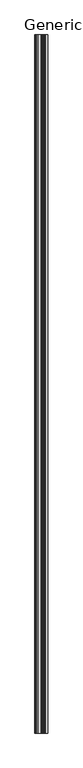
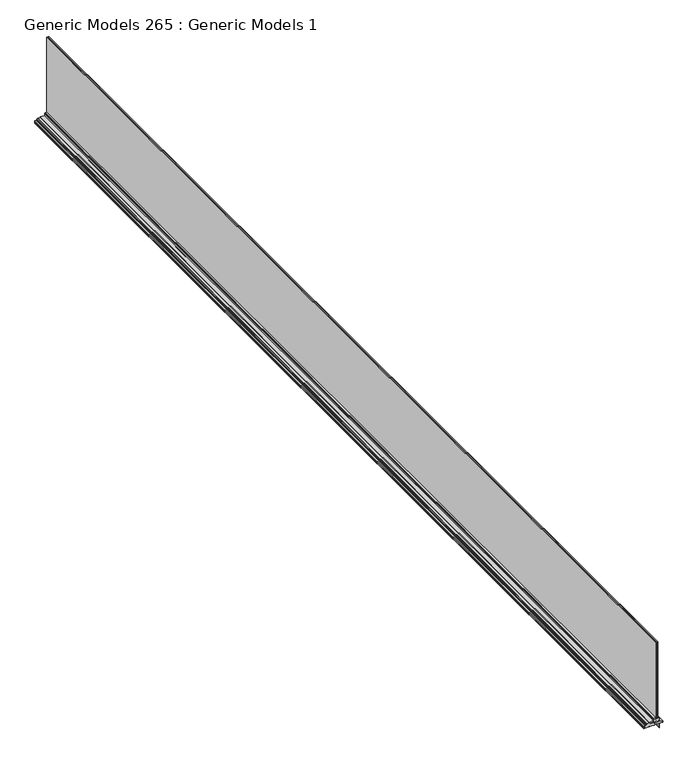
"""IFC4 building model written with IfcOpenShell, lengths in millimetres: proxy geometry, Generic Models 265 : Generic Models 1."""

from ifc_helpers import new_model, si_unit, point, frame, frame_2d, origin, place, context, project, spatial, polyline, circle_curve, trimmed, segment, composite_curve, outline, extrude, source, transform, mapped, element, save


def generic_models_265_generic_models_1_5434f9f2(model_context):
    return source(origin(), model_context, "Body", "SweptSolid", [
        extrude(outline(composite_curve([segment(polyline([(125550.1321292, 1521.9214201), (125550.1321292, 1539.9899635), (125553.3071292, 1539.9899635), (125553.3071292, 1542.2759674), (125550.1321292, 1542.2759674), (125550.1321292, 1559.7837165), (125553.3071292, 1559.7837165), (125553.3071292, 1562.0697204), (125550.1321292, 1562.0697204), (125550.1321292, 1579.0968201), (125552.2149292, 1579.0968201), (125552.2149292, 1582.2718201), (125550.1321292, 1582.2718201), (125550.1321292, 1599.3712026), (125553.3071292, 1599.3712026), (125553.3071292, 1601.6572026), (125550.1321292, 1601.6572026), (125550.1321292, 1638.1263704), (125514.7602416, 1638.1263704)]), True, "CONTINUOUS"), segment(trimmed(circle_curve(frame_2d((125514.7625825, 1638.8248707)), 0.6985041), [point((125514.7602416, 1638.1263704))], [point((125514.7650422, 1639.5233704))], False, "CARTESIAN"), True, "CONTINUOUS"), segment(polyline([(125514.7650422, 1639.5233704), (125550.1321292, 1639.5233704), (125550.1321292, 1664.4112048), (125551.5291292, 1664.4112048), (125551.5291292, 1658.0612048), (125553.8151292, 1658.0612048), (125553.8151292, 1665.9647704), (125562.7465526, 1665.9647704), (125565.1689224, 1638.1009704), (125565.1689224, 1603.1505704), (125570.0457151, 1603.1505704), (125570.0457151, 1599.1374433), (125563.6267755, 1599.1374433), (125563.6267755, 1597.1561689), (125571.5769685, 1597.1561689), (125571.5769685, 1588.7488332), (125572.516765, 1588.7488332), (125572.516765, 1571.2228332), (125574.802765, 1571.2228332), (125574.802765, 1588.7488332), (125583.489565, 1588.7488332), (125583.489565, 1591.7968061), (125586.664565, 1591.7968061), (125586.664565, 1562.3835821), (125580.3327325, 1562.3835821), (125580.3327325, 1543.3335821), (125577.945136, 1543.3335821), (125577.945136, 1541.7333891), (125574.770136, 1537.7964201), (125574.770136, 1536.196227), (125570.8077325, 1536.196227), (125570.8077325, 1533.021227), (125569.994943, 1532.2337751), (125569.994943, 1521.9214201), (125560.063524, 1521.9214201), (125560.063524, 1529.8716131), (125558.0823465, 1529.8716131), (125558.0823465, 1521.9214201), (125550.1321292, 1521.9214201)]), True, "CONTINUOUS")], self_intersect=False)), frame((0.0, 306.6963299, 0.0), z_axis=(0.0, 1.0, 0.0), x_axis=(0.0, 0.0, 1.0)), (0.0, 0.0, 1.0), 7886.7),
        extrude(outline(composite_curve([segment(polyline([(125598.9890401, 1629.6245125), (125597.965898, 1628.6013704), (125594.3852792, 1628.6013704), (125594.3852792, 1607.1639996), (125596.773568, 1609.5522884), (125606.704968, 1609.5522884), (125605.692318, 1597.724608), (125603.529968, 1597.724608), (125603.529968, 1593.9566884), (125595.986168, 1593.9566884), (125595.986168, 1595.5568884), (125594.3852792, 1595.5568884), (125594.3852792, 1593.6763704), (125576.0972792, 1593.6763704)]), True, "CONTINUOUS"), segment(trimmed(circle_curve(frame_2d((125576.0972792, 1594.4891704)), 0.8128), [point((125576.0972792, 1593.6763704))], [point((125575.2844792, 1594.4891704))], False, "CARTESIAN"), True, "CONTINUOUS"), segment(polyline([(125575.2844792, 1594.4891704), (125575.2844792, 1607.8241704)]), True, "CONTINUOUS"), segment(trimmed(circle_curve(frame_2d((125575.2844792, 1609.8053704)), 1.9812), [point((125575.2844792, 1607.8241704))], [point((125575.2844792, 1611.7865704))], True, "CARTESIAN"), True, "CONTINUOUS"), segment(polyline([(125575.2844792, 1611.7865704), (125575.2844792, 1623.9785704), (125569.9758792, 1623.9785704), (125569.9758792, 1629.5919704), (125577.9006792, 1629.5919704), (125577.9006792, 1631.4969704), (125574.5986792, 1631.4969704), (125574.5986792, 1633.1733704), (125572.5666792, 1633.1733704), (125572.5666792, 1635.7387704)]), True, "CONTINUOUS"), segment(trimmed(circle_curve(frame_2d((125574.9542792, 1635.7387704)), 2.3876), [point((125572.5666792, 1635.7387704))], [point((125574.9542792, 1638.1263704))], False, "CARTESIAN"), True, "CONTINUOUS"), segment(polyline([(125574.9542792, 1638.1263704), (125597.2554792, 1638.1263704), (125597.2554792, 1635.7387704), (125605.0613027, 1633.2034099), (125605.2508531, 1630.7603704), (125603.2244792, 1630.7603704), (125603.2244792, 1629.6245125), (125598.9890401, 1629.6245125)]), True, "CONTINUOUS")], self_intersect=False)), frame((0.0, 306.6963299, 0.0), z_axis=(0.0, 1.0, 0.0), x_axis=(0.0, 0.0, 1.0)), (0.0, 0.0, 1.0), 7886.7),
        extrude(outline(polyline([(1615.1085384, 306.6963299), (1610.3460384, 306.6963299), (1610.3460384, 8193.3963299), (1615.1085384, 8193.3963299), (1615.1085384, 306.6963299)])), frame((0.0, 0.0, 125595.1790292), z_axis=(0.0, 0.0, 1.0), x_axis=(1.0, 0.0, 0.0)), (0.0, 0.0, 1.0), 602.3375481),
        extrude(outline(polyline([(1622.2513704, 306.6963299), (1615.9022884, 306.6963299), (1615.9022884, 8193.3963299), (1622.2513704, 8193.3963299), (1622.2513704, 306.6963299)])), frame((0.0, 0.0, 125595.1790292), z_axis=(0.0, 0.0, 1.0), x_axis=(1.0, 0.0, 0.0)), (0.0, 0.0, 1.0), 6.35),
        extrude(outline(polyline([(1627.8076204, 306.6963299), (1623.0451204, 306.6963299), (1623.0451204, 8193.3963299), (1627.8076204, 8193.3963299), (1627.8076204, 306.6963299)])), frame((0.0, 0.0, 125595.1790292), z_axis=(0.0, 0.0, 1.0), x_axis=(1.0, 0.0, 0.0)), (0.0, 0.0, 1.0), 602.3375481),
    ])


if __name__ == "__main__":
    model = new_model("IFC4")
    model_context = context("Model", 3, world=origin())
    ifc_project = project(units=[si_unit("LENGTHUNIT", "METRE", prefix="MILLI")], contexts=[model_context])
    site = spatial("IfcSite", under=ifc_project)
    building = spatial("IfcBuilding", under=site)
    placement = place(None, origin())
    generic_models_265_generic_models_1_shape = generic_models_265_generic_models_1_5434f9f2(model_context)
    element("IfcBuildingElementProxy", 1, Name="Generic Models 265 : Generic Models 1", ObjectType="Generic Models 265 : Generic Models 1", at=placement, inside=building, context=model_context, shape_type="MappedRepresentation", body=[
        mapped(generic_models_265_generic_models_1_shape, transform((0.0, 0.0, 0.0), x_axis=(1.0, 0.0, 0.0), y_axis=(0.0, 1.0, 0.0), z_axis=(0.0, 0.0, 1.0))),
    ])
    save(model, "model.ifc")

# Revit data of these elements
# Element 1 (IfcBuildingElementProxy, "Generic Models 265 : Generic Models 1")
#   Materials on its faces: "_WINDOW PER SCHEDULE"
# Materials
#   "_WINDOW PER SCHEDULE": class "Generic", colour RGB 255 255 255, transparency 0, Cost = 0
